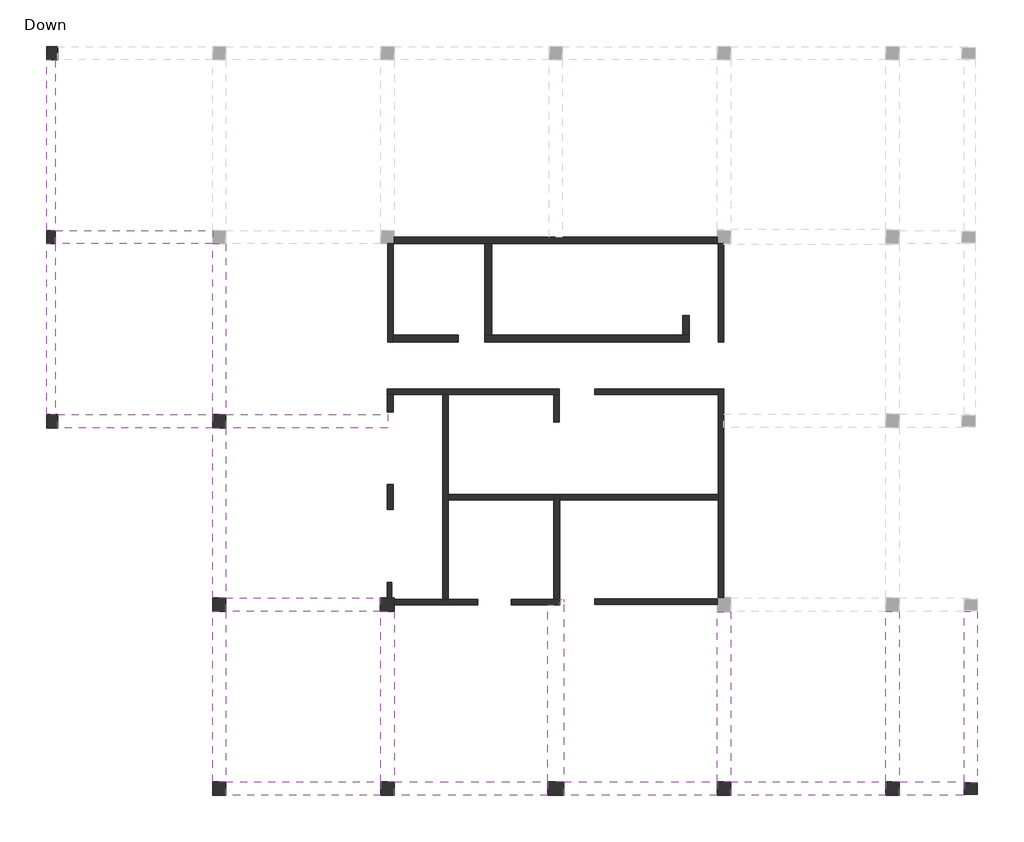
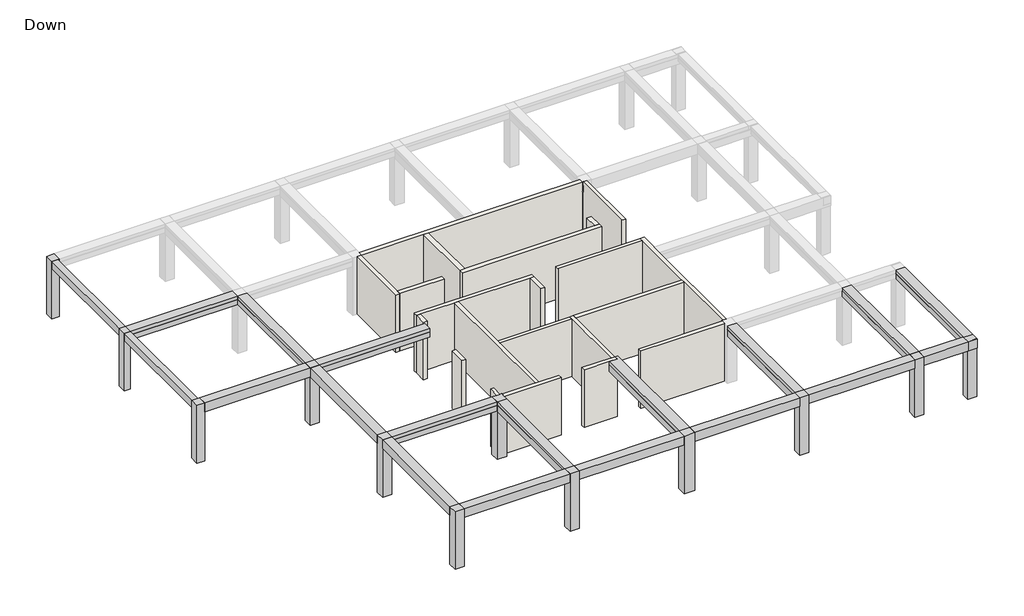
# One storey, part 1 of 2: 21 walls, 19 beams, 12 columns.
# Revit data of these elements (continued)
# Element 35 (IfcWall, "25") (continued)
#   SOFiSTiK_EdgeZones = "W7"
#   SOFiSTiK_AMG_Comments = ""
#   Top Offset = 0 cm
#   Base Offset = 0 cm
#   Unconnected Height = 400 cm
#   wall height = 400 cm
#   SOFiSTiK_AMG_Scheduled = yes
#   SOFiSTiK_AMG_Adjusted = yes
#   Phase Created = New Construction
#   Base Constraint = Down
#   Top Constraint = Typical Floor
#   Materials on its faces: "Concrete"
# Element 36 (IfcWall, "25")
#   Comments = ""
#   Mark = "W8"
#   SOFiSTiK_EdgeZones = "W8"
#   SOFiSTiK_AMG_Comments = ""
#   Top Offset = 0 cm
#   Base Offset = 0 cm
#   Unconnected Height = 400 cm
#   wall height = 400 cm
#   SOFiSTiK_AMG_Scheduled = yes
#   SOFiSTiK_AMG_Adjusted = yes
#   Phase Created = New Construction
#   Base Constraint = Down
#   Top Constraint = Typical Floor
#   Materials on its faces: "Concrete"
# Element 37 (IfcWall, "25")
#   Comments = ""
#   Mark = "W9"
#   SOFiSTiK_EdgeZones = "W9"
#   SOFiSTiK_AMG_Comments = ""
#   Top Offset = 0 cm
#   Base Offset = 0 cm
#   Unconnected Height = 400 cm
#   wall height = 400 cm
#   SOFiSTiK_AMG_Scheduled = yes
#   SOFiSTiK_AMG_Adjusted = yes
#   Phase Created = New Construction
#   Base Constraint = Down
#   Top Constraint = Typical Floor
#   Materials on its faces: "Concrete"
# Element 38 (IfcWall, "25")
#   Comments = ""
#   Mark = "W10"
#   SOFiSTiK_EdgeZones = "W10"
#   SOFiSTiK_AMG_Comments = ""
#   Top Offset = 0 cm
#   Base Offset = 0 cm
#   Unconnected Height = 400 cm
#   wall height = 400 cm
#   SOFiSTiK_AMG_Scheduled = yes
#   SOFiSTiK_AMG_Adjusted = yes
#   Phase Created = New Construction
#   Base Constraint = Down
#   Top Constraint = Typical Floor
#   Materials on its faces: "Concrete"
# Element 39 (IfcWall, "25")
#   Comments = ""
#   Mark = "W11"
#   SOFiSTiK_EdgeZones = "W11"
#   SOFiSTiK_AMG_Comments = ""
#   Top Offset = 0 cm
#   Base Offset = 0 cm
#   Unconnected Height = 400 cm
#   wall height = 400 cm
#   SOFiSTiK_AMG_Scheduled = yes
#   SOFiSTiK_AMG_Adjusted = yes
#   Phase Created = New Construction
#   Base Constraint = Down
#   Top Constraint = Typical Floor
#   Materials on its faces: "Concrete"
# Element 40 (IfcWall, "25")
#   Comments = ""
#   Mark = "W12"
#   SOFiSTiK_EdgeZones = "W12"
#   SOFiSTiK_AMG_Comments = ""
#   Top Offset = 0 cm
#   Base Offset = 0 cm
#   Unconnected Height = 400 cm
#   wall height = 400 cm
#   SOFiSTiK_AMG_Scheduled = yes
#   SOFiSTiK_AMG_Adjusted = yes
#   Phase Created = New Construction
#   Base Constraint = Down
#   Top Constraint = Typical Floor
#   Materials on its faces: "Concrete"
# Element 41 (IfcWall, "25")
#   Comments = ""
#   Mark = "W13"
#   SOFiSTiK_EdgeZones = "W13"
#   SOFiSTiK_AMG_Comments = ""
#   Top Offset = 0 cm
#   Base Offset = 0 cm
#   Unconnected Height = 400 cm
#   wall height = 400 cm
#   SOFiSTiK_AMG_Scheduled = yes
#   SOFiSTiK_AMG_Adjusted = yes
#   Phase Created = New Construction
#   Base Constraint = Down
#   Top Constraint = Typical Floor
#   Materials on its faces: "Concrete"
# Element 42 (IfcWall, "25")
#   Comments = ""
#   Mark = "W14"
#   SOFiSTiK_EdgeZones = "W14"
#   SOFiSTiK_AMG_Comments = ""
#   Top Offset = 0 cm
#   Base Offset = 0 cm
#   Unconnected Height = 400 cm
#   wall height = 400 cm
#   SOFiSTiK_AMG_Scheduled = yes
#   SOFiSTiK_AMG_Adjusted = yes
#   Phase Created = New Construction
#   Base Constraint = Down
#   Top Constraint = Typical Floor
#   Materials on its faces: "Concrete"
# Element 43 (IfcWall, "25")
#   Comments = ""
#   Mark = "W15"
#   SOFiSTiK_EdgeZones = "W15"
#   SOFiSTiK_AMG_Comments = ""
#   Top Offset = 0 cm
#   Base Offset = 0 cm
#   Unconnected Height = 400 cm
#   wall height = 400 cm
#   SOFiSTiK_AMG_Scheduled = yes
#   SOFiSTiK_AMG_Adjusted = yes
#   Phase Created = New Construction
#   Base Constraint = Down
#   Top Constraint = Typical Floor
#   Materials on its faces: "Concrete"
# Element 44 (IfcWall, "25")
#   Comments = ""
#   Mark = "W16"
#   SOFiSTiK_EdgeZones = "W16"
#   SOFiSTiK_AMG_Comments = ""
#   Top Offset = 0 cm
#   Base Offset = 0 cm
#   Unconnected Height = 400 cm
#   wall height = 400 cm
#   SOFiSTiK_AMG_Scheduled = yes
#   SOFiSTiK_AMG_Adjusted = yes
#   Phase Created = New Construction
#   Base Constraint = Down
#   Top Constraint = Typical Floor
#   Materials on its faces: "Concrete"
# Element 45 (IfcWall, "25")
#   Comments = ""
#   Mark = "W17"
#   SOFiSTiK_EdgeZones = "W17"
#   SOFiSTiK_AMG_Comments = ""
#   Top Offset = 0 cm
#   Base Offset = 0 cm
#   Unconnected Height = 400 cm
#   wall height = 400 cm
#   SOFiSTiK_AMG_Scheduled = yes
#   SOFiSTiK_AMG_Adjusted = yes
#   Phase Created = New Construction
#   Base Constraint = Down
#   Top Constraint = Typical Floor
#   Materials on its faces: "Concrete"
# Element 46 (IfcWall, "25")
#   Comments = ""
#   Mark = "W18"
#   SOFiSTiK_EdgeZones = "W18"
#   SOFiSTiK_AMG_Comments = ""
#   Top Offset = 0 cm
#   Base Offset = 0 cm
#   Unconnected Height = 400 cm
#   wall height = 400 cm
#   SOFiSTiK_AMG_Scheduled = yes
#   SOFiSTiK_AMG_Adjusted = yes
#   Phase Created = New Construction
#   Base Constraint = Down
#   Top Constraint = Typical Floor
#   Materials on its faces: "Concrete"
# Element 47 (IfcWall, "25")
#   Comments = ""
#   Mark = "W19"
#   SOFiSTiK_EdgeZones = "W19"
#   SOFiSTiK_AMG_Comments = ""
#   Top Offset = 0 cm
#   Base Offset = 0 cm
#   Unconnected Height = 400 cm
#   wall height = 400 cm
#   SOFiSTiK_AMG_Scheduled = yes
#   SOFiSTiK_AMG_Adjusted = yes
#   Phase Created = New Construction
#   Base Constraint = Down
#   Top Constraint = Typical Floor
#   Materials on its faces: "Concrete"
# Element 48 (IfcWall, "30")
#   Comments = ""
#   Mark = "W1"
#   SOFiSTiK_EdgeZones = "W1"
#   SOFiSTiK_AMG_Comments = ""
#   Top Offset = 0 cm
#   Base Offset = 0 cm
#   Unconnected Height = 400 cm
#   wall height = 400 cm
#   SOFiSTiK_AMG_Scheduled = yes
#   SOFiSTiK_AMG_Adjusted = yes
#   Phase Created = New Construction
#   Base Constraint = Down
#   Top Constraint = Typical Floor
#   Materials on its faces: "Concrete"
# Element 49 (IfcWall, "30")
#   Comments = ""
#   Mark = "W2"
#   SOFiSTiK_EdgeZones = "W2"
#   SOFiSTiK_AMG_Comments = ""
#   Top Offset = 0 cm
#   Base Offset = 0 cm
#   Unconnected Height = 400 cm
#   wall height = 400 cm
#   SOFiSTiK_AMG_Scheduled = yes
#   SOFiSTiK_AMG_Adjusted = yes
#   Phase Created = New Construction
#   Base Constraint = Down
#   Top Constraint = Typical Floor
#   Materials on its faces: "Concrete"
# Element 50 (IfcWall, "30")
#   Comments = ""
#   Mark = "W3"
#   SOFiSTiK_EdgeZones = "W3"
#   SOFiSTiK_AMG_Comments = ""
#   Top Offset = 0 cm
#   Base Offset = 0 cm
#   Unconnected Height = 400 cm
#   wall height = 400 cm
#   SOFiSTiK_AMG_Scheduled = yes
#   SOFiSTiK_AMG_Adjusted = yes
#   Phase Created = New Construction
#   Base Constraint = Down
#   Top Constraint = Typical Floor
#   Materials on its faces: "Concrete"
# Element 51 (IfcWall, "30")
#   Comments = ""
#   Mark = "W4"
#   SOFiSTiK_EdgeZones = "W4"
#   SOFiSTiK_AMG_Comments = ""
#   Top Offset = 0 cm
#   Base Offset = 0 cm
#   Unconnected Height = 400 cm
#   wall height = 400 cm
#   SOFiSTiK_AMG_Scheduled = yes
#   SOFiSTiK_AMG_Adjusted = yes
#   Phase Created = New Construction
#   Base Constraint = Down
#   Top Constraint = Typical Floor
#   Materials on its faces: "Concrete"
# Element 52 (IfcWall, "33")
#   Comments = ""
#   Mark = "W20"
#   SOFiSTiK_EdgeZones = "W20"
#   SOFiSTiK_AMG_Comments = ""
#   Top Offset = 0 cm
#   Base Offset = 0 cm
#   Unconnected Height = 400 cm
#   wall height = 400 cm
#   SOFiSTiK_AMG_Scheduled = yes
#   SOFiSTiK_AMG_Adjusted = yes
#   Phase Created = New Construction
#   Base Constraint = Down
#   Top Constraint = Typical Floor
#   Materials on its faces: "Concrete"
# Materials
#   "Concrete": class "Concrete", colour RGB 192 192 192, transparency 0, Keynote = "01000", Description = "Cast-in-place concrete", Cost = 0
